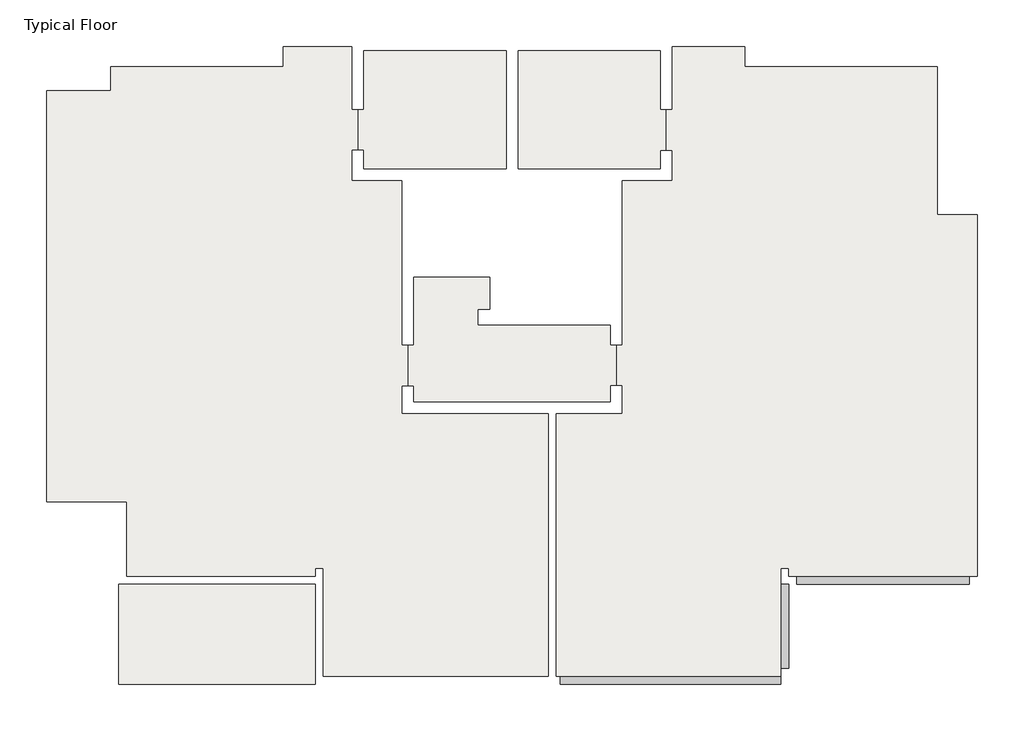
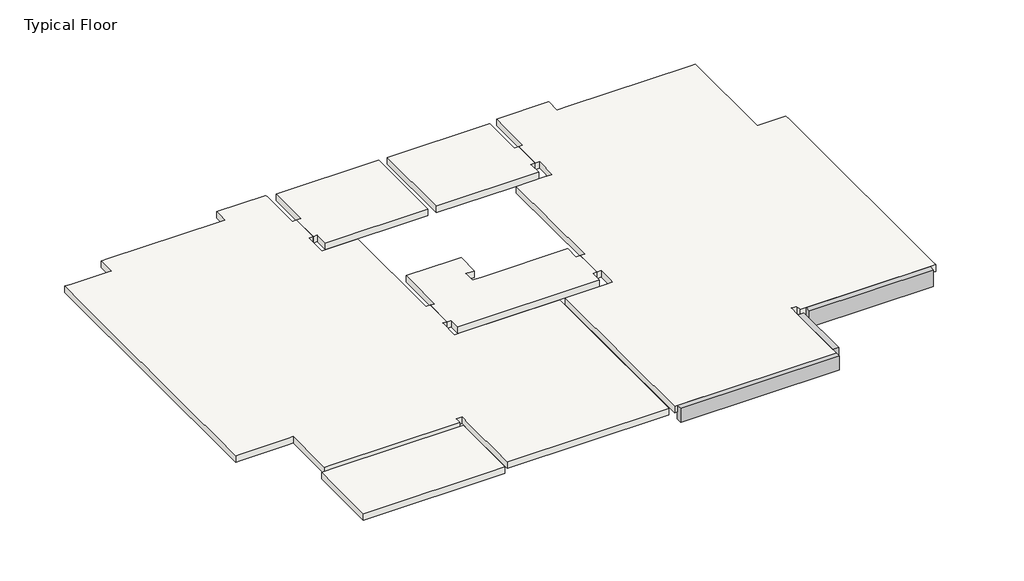
# One storey: 6 slabs, 3 beams.
"""IFC4 building model written with IfcOpenShell, lengths in millimetres."""

from ifc_helpers import new_model, si_unit, frame, origin, place, context, project, spatial, polyline, outline, extrude, faceted_brep, element, save

model = new_model("IFC4")

# Units and contexts
model_context = context("Model", 3, world=origin())
ifc_project = project(units=[si_unit("LENGTHUNIT", "METRE", prefix="MILLI")], contexts=[model_context])

# Site, building, storey
site = spatial("IfcSite", under=ifc_project)
building = spatial("IfcBuilding", under=site)
storey = spatial("IfcBuildingStorey", under=building, Name="Typical Floor", Elevation=3100.0)

# Beams
placement = place(None, origin())
element("IfcBeam", 1, ObjectType="Concrete Rectengular Beam : 20/50", at=placement, inside=storey, context=model_context, shape_type="Brep", body=[
    faceted_brep([(6304.7124885, -12504.8386239, 3100.0), (6304.7124885, -12304.8386239, 3100.0), (804.183388, -12304.8386239, 3100.0), (804.183388, -12504.8386239, 3100.0), (6304.7124885, -12304.8386239, 2860.0), (6304.7124885, -12304.8386239, 2600.0), (804.183388, -12304.8386239, 2600.0), (6304.7124885, -12504.8386239, 2600.0), (804.183388, -12504.8386239, 2600.0)], [[[0, 1, 2, 3]], [[1, 4, 5, 6, 2]], [[5, 7, 8, 6]], [[3, 8, 7, 0]], [[0, 7, 5, 4, 1]], [[3, 2, 6, 8]]]),
])
element("IfcBeam", 2, ObjectType="Concrete Rectengular Beam : 20/60", at=placement, inside=storey, context=model_context, shape_type="Brep", body=[
    faceted_brep([(6704.7124885, -9805.3677244, 3100.0), (6704.7124885, -10005.3677244, 3100.0), (11003.1251869, -10005.3677244, 3100.0), (11003.1251869, -9805.3677244, 3100.0), (6704.7124885, -10005.3677244, 2500.0), (11003.1251869, -10005.3677244, 2500.0), (6704.7124885, -9805.3677244, 2500.0), (11003.1251869, -9805.3677244, 2500.0), (11003.1251869, -9805.3677244, 2860.0), (6704.7124885, -9805.3677244, 2860.0)], [[[0, 1, 2, 3]], [[1, 4, 5, 2]], [[4, 6, 7, 5]], [[0, 3, 8, 7, 6, 9]], [[1, 0, 9, 6, 4]], [[3, 2, 5, 7, 8]]]),
])
element("IfcBeam", 3, ObjectType="Concrete Rectengular Beam : 20/60", at=placement, inside=storey, context=model_context, shape_type="Brep", body=[
    faceted_brep([(6304.7124885, -12104.8386239, 3100.0), (6504.7124885, -12104.8386239, 3100.0), (6504.7124885, -10005.3677244, 3100.0), (6304.7124885, -10005.3677244, 3100.0), (6504.7124885, -12104.8386239, 2500.0), (6504.7124885, -10005.3677244, 2500.0), (6304.7124885, -12104.8386239, 2500.0), (6304.7124885, -10005.3677244, 2500.0), (6304.7124885, -10005.3677244, 2860.0), (6304.7124885, -12104.8386239, 2860.0)], [[[0, 1, 2, 3]], [[1, 4, 5, 2]], [[4, 6, 7, 5]], [[0, 3, 8, 7, 6, 9]], [[1, 0, 9, 6, 4]], [[2, 5, 7, 8, 3]]]),
])

# Slabs
element("IfcSlab", 4, ObjectType="24", at=placement, inside=storey, context=model_context, shape_type="Brep", body=[
    faceted_brep([(2051.273335, -4056.1613752, 2860.0), (2201.273335, -4056.1613752, 2860.0), (2201.273335, -5055.6322747, 2860.0), (2053.3897372, -5055.6322747, 2860.0), (2053.3897372, -5455.6322747, 2860.0), (-2847.1393634, -5455.6322747, 2860.0), (-2847.1393634, -5057.2195763, 2860.0), (-2997.1393634, -5057.2195763, 2860.0), (-2997.1393634, -4056.1613752, 2860.0), (-2847.1393634, -4056.1613752, 2860.0), (-2847.1393634, -2356.6904757, 2860.0), (-1246.6102628, -2356.6904757, 2860.0), (-946.6102628, -2356.6904757, 2860.0), (-946.6102628, -3156.6904757, 2860.0), (-1246.6102628, -3156.6904757, 2860.0), (-1246.6102628, -3556.6904757, 2860.0), (-946.6102628, -3556.6904757, 2860.0), (2051.273335, -3556.6904757, 2860.0), (2201.273335, -4056.1613752, 3100.0), (2051.273335, -4056.1613752, 3100.0), (2051.273335, -3556.6904757, 3100.0), (-946.6102628, -3556.6904757, 3100.0), (-1246.6102628, -3556.6904757, 3100.0), (-1246.6102628, -3156.6904757, 3100.0), (-946.6102628, -3156.6904757, 3100.0), (-946.6102628, -2356.6904757, 3100.0), (-1246.6102628, -2356.6904757, 3100.0), (-2847.1393634, -2356.6904757, 3100.0), (-2847.1393634, -4056.1613752, 3100.0), (-2997.1393634, -4056.1613752, 3100.0), (-2997.1393634, -5057.2195763, 3100.0), (-2847.1393634, -5057.2195763, 3100.0), (-2847.1393634, -5455.6322747, 3100.0), (2053.3897372, -5455.6322747, 3100.0), (2053.3897372, -5055.6322747, 3100.0), (2201.273335, -5055.6322747, 3100.0)], [[[0, 1, 2, 3, 4, 5, 6, 7, 8, 9, 10, 11, 12, 13, 14, 15, 16, 17]], [[18, 19, 20, 21, 22, 23, 24, 25, 26, 27, 28, 29, 30, 31, 32, 33, 34, 35]], [[1, 0, 19, 18]], [[2, 1, 18, 35]], [[3, 2, 35, 34]], [[4, 3, 34, 33]], [[5, 4, 33, 32]], [[6, 5, 32, 31]], [[7, 6, 31, 30]], [[8, 7, 30, 29]], [[9, 8, 29, 28]], [[10, 9, 28, 27]], [[11, 10, 27, 26]], [[12, 11, 26, 25]], [[13, 12, 25, 24]], [[14, 13, 24, 23]], [[15, 14, 23, 22]], [[15, 22, 21, 20, 17, 16]], [[0, 17, 20, 19]]]),
])
element("IfcSlab", 5, ObjectType="24", at=placement, inside=storey, context=model_context, shape_type="SweptSolid", body=[
    extrude(outline(polyline([(3302.0669858, 3291.4576724), (3302.0669858, 1816.8544978), (3452.0669858, 1816.8544978), (3452.0669858, 811.5634925), (3302.0669858, 811.5634925), (3302.0669858, 343.3095243), (-246.0811623, 343.3095243), (-246.0811623, 3291.4576724), (3302.0669858, 3291.4576724)])), frame((0.0, 0.0, 2860.0), z_axis=(0.0, 0.0, 1.0), x_axis=(1.0, 0.0, 0.0)), (0.0, 0.0, 1.0), 240.0),
])
element("IfcSlab", 6, ObjectType="24", at=placement, inside=storey, context=model_context, shape_type="SweptSolid", body=[
    extrude(outline(polyline([(-546.0811623, 3291.4576724), (-546.0811623, 343.3095243), (-4095.816612, 343.3095243), (-4095.816612, 817.9126989), (-4245.816612, 817.9126989), (-4245.816612, 1816.8544978), (-4095.816612, 1816.8544978), (-4095.816612, 3291.4576724), (-546.0811623, 3291.4576724)])), frame((0.0, 0.0, 2860.0), z_axis=(0.0, 0.0, 1.0), x_axis=(1.0, 0.0, 0.0)), (0.0, 0.0, 1.0), 240.0),
])
element("IfcSlab", 7, ObjectType="24", at=placement, inside=storey, context=model_context, shape_type="Brep", body=[
    faceted_brep([(3452.0669858, 1816.8544978, 2860.0), (3602.0669858, 1816.8544978, 2860.0), (3602.0669858, 3291.4576724, 2860.0), (3602.0669858, 3391.4576724, 2860.0), (5403.1251869, 3391.4576724, 2860.0), (5403.1251869, 2891.9867729, 2860.0), (5803.1251869, 2891.9867729, 2860.0), (10002.0669858, 2891.9867729, 2860.0), (10202.0669858, 2891.9867729, 2860.0), (10202.0669858, 2691.9867729, 2860.0), (10202.0669858, -606.4259255, 2860.0), (10202.0669858, -806.4259255, 2860.0), (11203.1251869, -806.4259255, 2860.0), (11203.1251869, -9605.3677244, 2860.0), (11203.1251869, -9805.3677244, 2860.0), (11003.1251869, -9805.3677244, 2860.0), (6704.7124885, -9805.3677244, 2860.0), (6504.7124885, -9805.3677244, 2860.0), (6504.7124885, -9605.3677244, 2860.0), (6304.7124885, -9605.3677244, 2860.0), (6304.7124885, -10005.3677244, 2860.0), (6304.7124885, -12104.8386239, 2860.0), (6304.7124885, -12304.8386239, 2860.0), (804.183388, -12304.8386239, 2860.0), (704.183388, -12304.8386239, 2860.0), (704.183388, -12104.8386239, 2860.0), (704.183388, -5755.6322747, 2860.0), (2053.3897372, -5755.6322747, 2860.0), (2353.3897372, -5755.6322747, 2860.0), (2353.3897372, -5055.6322747, 2860.0), (2203.3897372, -5055.6322747, 2860.0), (2201.273335, -5055.6322747, 2860.0), (2201.273335, -4056.1613752, 2860.0), (2351.273335, -4056.1613752, 2860.0), (2351.273335, 43.3095243, 2860.0), (3302.0669858, 43.3095243, 2860.0), (3602.0669858, 43.3095243, 2860.0), (3602.0669858, 811.5634925, 2860.0), (3452.0669858, 811.5634925, 2860.0), (3602.0669858, 1816.8544978, 3100.0), (3452.0669858, 1816.8544978, 3100.0), (3452.0669858, 811.5634925, 3100.0), (3602.0669858, 811.5634925, 3100.0), (3602.0669858, 43.3095243, 3100.0), (3302.0669858, 43.3095243, 3100.0), (2351.273335, 43.3095243, 3100.0), (2351.273335, -4056.1613752, 3100.0), (2201.273335, -4056.1613752, 3100.0), (2201.273335, -5055.6322747, 3100.0), (2203.3897372, -5055.6322747, 3100.0), (2353.3897372, -5055.6322747, 3100.0), (2353.3897372, -5755.6322747, 3100.0), (2053.3897372, -5755.6322747, 3100.0), (704.183388, -5755.6322747, 3100.0), (704.183388, -9405.3677244, 3100.0), (704.183388, -10005.3677244, 3100.0), (704.183388, -12104.8386239, 3100.0), (704.183388, -12304.8386239, 3100.0), (804.183388, -12304.8386239, 3100.0), (6304.7124885, -12304.8386239, 3100.0), (6304.7124885, -12104.8386239, 3100.0), (6304.7124885, -10005.3677244, 3100.0), (6304.7124885, -9605.3677244, 3100.0), (6504.7124885, -9605.3677244, 3100.0), (6504.7124885, -9805.3677244, 3100.0), (6704.7124885, -9805.3677244, 3100.0), (11003.1251869, -9805.3677244, 3100.0), (11203.1251869, -9805.3677244, 3100.0), (11203.1251869, -9605.3677244, 3100.0), (11203.1251869, -5956.955026, 3100.0), (11203.1251869, -5306.955026, 3100.0), (11203.1251869, -1006.4259255, 3100.0), (11203.1251869, -806.4259255, 3100.0), (10202.0669858, -806.4259255, 3100.0), (10202.0669858, -606.4259255, 3100.0), (10202.0669858, 2691.9867729, 3100.0), (10202.0669858, 2891.9867729, 3100.0), (10002.0669858, 2891.9867729, 3100.0), (5803.1251869, 2891.9867729, 3100.0), (5403.1251869, 2891.9867729, 3100.0), (5403.1251869, 3391.4576724, 3100.0), (3602.0669858, 3391.4576724, 3100.0), (3602.0669858, 3291.4576724, 3100.0)], [[[0, 1, 2, 3, 4, 5, 6, 7, 8, 9, 10, 11, 12, 13, 14, 15, 16, 17, 18, 19, 20, 21, 22, 23, 24, 25, 26, 27, 28, 29, 30, 31, 32, 33, 34, 35, 36, 37, 38]], [[39, 40, 41, 42, 43, 44, 45, 46, 47, 48, 49, 50, 51, 52, 53, 54, 55, 56, 57, 58, 59, 60, 61, 62, 63, 64, 65, 66, 67, 68, 69, 70, 71, 72, 73, 74, 75, 76, 77, 78, 79, 80, 81, 82]], [[1, 0, 40, 39]], [[1, 39, 82, 81, 3, 2]], [[4, 3, 81, 80]], [[5, 4, 80, 79]], [[5, 79, 78, 77, 76, 8, 7, 6]], [[8, 76, 75, 74, 73, 11, 10, 9]], [[12, 11, 73, 72]], [[12, 72, 71, 70, 69, 68, 67, 14, 13]], [[14, 67, 66, 65, 64, 17, 16, 15]], [[18, 17, 64, 63]], [[19, 18, 63, 62]], [[20, 19, 62, 61]], [[20, 61, 60, 59, 22, 21]], [[22, 59, 58, 57, 24, 23]], [[24, 57, 56, 55, 54, 53, 26, 25]], [[26, 53, 52, 51, 28, 27]], [[29, 28, 51, 50]], [[30, 29, 50, 49]], [[31, 30, 49, 48]], [[32, 31, 48, 47]], [[33, 32, 47, 46]], [[34, 33, 46, 45]], [[34, 45, 44, 43, 36, 35]], [[37, 36, 43, 42]], [[38, 37, 42, 41]], [[0, 38, 41, 40]]]),
])
element("IfcSlab", 8, ObjectType="24", at=placement, inside=storey, context=model_context, shape_type="Brep", body=[
    faceted_brep([(-5097.4039136, -9605.3677244, 2860.0), (-5297.4039136, -9605.3677244, 2860.0), (-5297.4039136, -9805.3677244, 2860.0), (-5497.4039136, -9805.3677244, 2860.0), (-9695.2875115, -9805.3677244, 2860.0), (-9995.816612, -9805.3677244, 2860.0), (-9995.816612, -7955.6322747, 2860.0), (-10195.816612, -7955.6322747, 2860.0), (-11796.8748131, -7955.6322747, 2860.0), (-11996.8748131, -7955.6322747, 2860.0), (-11996.8748131, -7755.6322747, 2860.0), (-11996.8748131, 2091.9867729, 2860.0), (-11996.8748131, 2291.9867729, 2860.0), (-11796.8748131, 2291.9867729, 2860.0), (-10596.8748131, 2291.9867729, 2860.0), (-10396.8748131, 2291.9867729, 2860.0), (-10396.8748131, 2891.9867729, 2860.0), (-10196.8748131, 2891.9867729, 2860.0), (-6296.3457126, 2891.9867729, 2860.0), (-6096.3457126, 2891.9867729, 2860.0), (-6096.3457126, 3391.4576724, 2860.0), (-4395.816612, 3391.4576724, 2860.0), (-4395.816612, 3291.4576724, 2860.0), (-4395.816612, 1816.8544978, 2860.0), (-4245.816612, 1816.8544978, 2860.0), (-4245.816612, 817.9126989, 2860.0), (-4395.816612, 817.9126989, 2860.0), (-4395.816612, 343.3095243, 2860.0), (-4395.816612, 43.3095243, 2860.0), (-3147.1393634, 43.3095243, 2860.0), (-3147.1393634, -4056.1613752, 2860.0), (-2997.1393634, -4056.1613752, 2860.0), (-2997.1393634, -5057.2195763, 2860.0), (-3147.1393634, -5057.2195763, 2860.0), (-3147.1393634, -5755.6322747, 2860.0), (-2847.1393634, -5755.6322747, 2860.0), (504.183388, -5755.6322747, 2860.0), (504.183388, -12104.8386239, 2860.0), (504.183388, -12304.8386239, 2860.0), (404.183388, -12304.8386239, 2860.0), (-5097.4039136, -12304.8386239, 2860.0), (-5097.4039136, -12104.8386239, 2860.0), (-5097.4039136, -10005.3677244, 2860.0), (-5297.4039136, -9605.3677244, 3100.0), (-5097.4039136, -9605.3677244, 3100.0), (-5097.4039136, -10005.3677244, 3100.0), (-5097.4039136, -12104.8386239, 3100.0), (-5097.4039136, -12304.8386239, 3100.0), (404.183388, -12304.8386239, 3100.0), (504.183388, -12304.8386239, 3100.0), (504.183388, -12104.8386239, 3100.0), (504.183388, -10005.3677244, 3100.0), (504.183388, -9405.3677244, 3100.0), (504.183388, -5755.6322747, 3100.0), (-2847.1393634, -5755.6322747, 3100.0), (-3147.1393634, -5755.6322747, 3100.0), (-3147.1393634, -5057.2195763, 3100.0), (-2997.1393634, -5057.2195763, 3100.0), (-2997.1393634, -4056.1613752, 3100.0), (-3147.1393634, -4056.1613752, 3100.0), (-3147.1393634, 43.3095243, 3100.0), (-4395.816612, 43.3095243, 3100.0), (-4395.816612, 343.3095243, 3100.0), (-4395.816612, 817.9126989, 3100.0), (-4245.816612, 817.9126989, 3100.0), (-4245.816612, 1816.8544978, 3100.0), (-4395.816612, 1816.8544978, 3100.0), (-4395.816612, 3291.4576724, 3100.0), (-4395.816612, 3391.4576724, 3100.0), (-6096.3457126, 3391.4576724, 3100.0), (-6096.3457126, 2891.9867729, 3100.0), (-6296.3457126, 2891.9867729, 3100.0), (-10196.8748131, 2891.9867729, 3100.0), (-10396.8748131, 2891.9867729, 3100.0), (-10396.8748131, 2291.9867729, 3100.0), (-10596.8748131, 2291.9867729, 3100.0), (-11796.8748131, 2291.9867729, 3100.0), (-11996.8748131, 2291.9867729, 3100.0), (-11996.8748131, 2091.9867729, 3100.0), (-11996.8748131, -407.4841265, 3100.0), (-11996.8748131, -807.4841265, 3100.0), (-11996.8748131, -3806.4259255, 3100.0), (-11996.8748131, -4456.4259255, 3100.0), (-11996.8748131, -7755.6322747, 3100.0), (-11996.8748131, -7955.6322747, 3100.0), (-11796.8748131, -7955.6322747, 3100.0), (-10195.816612, -7955.6322747, 3100.0), (-9995.816612, -7955.6322747, 3100.0), (-9995.816612, -9805.3677244, 3100.0), (-9695.2875115, -9805.3677244, 3100.0), (-5497.4039136, -9805.3677244, 3100.0), (-5297.4039136, -9805.3677244, 3100.0)], [[[0, 1, 2, 3, 4, 5, 6, 7, 8, 9, 10, 11, 12, 13, 14, 15, 16, 17, 18, 19, 20, 21, 22, 23, 24, 25, 26, 27, 28, 29, 30, 31, 32, 33, 34, 35, 36, 37, 38, 39, 40, 41, 42]], [[43, 44, 45, 46, 47, 48, 49, 50, 51, 52, 53, 54, 55, 56, 57, 58, 59, 60, 61, 62, 63, 64, 65, 66, 67, 68, 69, 70, 71, 72, 73, 74, 75, 76, 77, 78, 79, 80, 81, 82, 83, 84, 85, 86, 87, 88, 89, 90, 91]], [[47, 40, 39, 38, 49, 48]], [[40, 47, 46, 45, 44, 0, 42, 41]], [[1, 0, 44, 43]], [[2, 1, 43, 91]], [[2, 91, 90, 89, 88, 5, 4, 3]], [[6, 5, 88, 87]], [[6, 87, 86, 85, 84, 9, 8, 7]], [[9, 84, 83, 82, 81, 80, 79, 78, 77, 12, 11, 10]], [[12, 77, 76, 75, 74, 15, 14, 13]], [[16, 15, 74, 73]], [[16, 73, 72, 71, 70, 19, 18, 17]], [[20, 19, 70, 69]], [[21, 20, 69, 68]], [[21, 68, 67, 66, 23, 22]], [[24, 23, 66, 65]], [[25, 24, 65, 64]], [[26, 25, 64, 63]], [[26, 63, 62, 61, 28, 27]], [[29, 28, 61, 60]], [[30, 29, 60, 59]], [[31, 30, 59, 58]], [[32, 31, 58, 57]], [[33, 32, 57, 56]], [[34, 33, 56, 55]], [[34, 55, 54, 53, 36, 35]], [[36, 53, 52, 51, 50, 49, 38, 37]]]),
])
element("IfcSlab", 9, ObjectType="24", at=placement, inside=storey, context=model_context, shape_type="Brep", body=[
    faceted_brep([(-5297.4039136, -10005.3677244, 2860.0), (-5297.4039136, -12504.8386239, 2860.0), (-10195.816612, -12504.8386239, 2860.0), (-10195.816612, -10005.3677244, 2860.0), (-5297.4039136, -12504.8386239, 3100.0), (-5297.4039136, -12104.8386239, 3100.0), (-5297.4039136, -10005.3677244, 3100.0), (-5497.4039136, -10005.3677244, 3100.0), (-9695.2875115, -10005.3677244, 3100.0), (-10195.816612, -10005.3677244, 3100.0), (-10195.816612, -12504.8386239, 3100.0)], [[[0, 1, 2, 3]], [[4, 5, 6, 7, 8, 9, 10]], [[1, 0, 6, 5, 4]], [[2, 1, 4, 10]], [[3, 2, 10, 9]], [[0, 3, 9, 8, 7, 6]]]),
])

save(model, "model.ifc")

# Revit data of these elements
# Type "Concrete Rectengular Beam : 20/50"
#   Length [instance default] = 152.4 cm
#   b = 20 cm
#   h = 50 cm
#   Structural Material [instance default] = Concrete
#   Assembly Code = ""
# Type "Concrete Rectengular Beam : 20/60"
#   Length [instance default] = 152.4 cm
#   b = 20 cm
#   h = 60 cm
#   Structural Material [instance default] = Concrete
#   Assembly Code = ""
# Type "24"
#   Function = 0
#   Layers, outside or top first: 24 cm "Concrete" (function 1)
# Element 1 (IfcBeam, "Concrete Rectengular Beam : 20/50")
#   Comments = ""
#   Mark = "B8"
#   SOFiSTiK_AMG_Comments = ""
#   SOFiSTiK_AMG_Scheduled = yes
#   SOFiSTiK_AMG_Adjusted = yes
#   Structural Material = Concrete
#   Phase Created = New Construction
#   Materials on its faces: "Concrete"
# Element 2 (IfcBeam, "Concrete Rectengular Beam : 20/60")
#   Comments = ""
#   Mark = "B19"
#   SOFiSTiK_AMG_Comments = ""
#   SOFiSTiK_AMG_Scheduled = yes
#   SOFiSTiK_AMG_Adjusted = yes
#   Structural Material = Concrete
#   Phase Created = New Construction
#   Materials on its faces: "Concrete"
# Element 3 (IfcBeam, "Concrete Rectengular Beam : 20/60")
#   Comments = ""
#   Mark = "B20"
#   SOFiSTiK_AMG_Comments = ""
#   SOFiSTiK_AMG_Scheduled = yes
#   SOFiSTiK_AMG_Adjusted = yes
#   Structural Material = Concrete
#   Phase Created = New Construction
#   Materials on its faces: "Concrete"
# Element 4 (IfcSlab, "24")
#   Mark = "S1"
#   SOFiSTiK_AMG_Comments = ""
#   built-in parameter 1001955 = -1.5708 (stored number, unit not read)
#   Height Offset From Level = 0 cm
#   built-in parameter 1001954 = 1
#   SOFiSTiK_AMG_Scheduled = yes
#   SOFiSTiK_AMG_Adjusted = yes
#   Phase Created = New Construction
#   Materials on its faces: "Concrete"
# Element 5 (IfcSlab, "24")
#   Mark = "S2"
#   SOFiSTiK_AMG_Comments = ""
#   Height Offset From Level = 0 cm
#   built-in parameter 1001954 = 1
#   SOFiSTiK_AMG_Scheduled = yes
#   SOFiSTiK_AMG_Adjusted = yes
#   Phase Created = New Construction
#   Materials on its faces: "Concrete"
# Element 6 (IfcSlab, "24")
#   Mark = "S3"
#   SOFiSTiK_AMG_Comments = ""
#   Height Offset From Level = 0 cm
#   built-in parameter 1001954 = 1
#   SOFiSTiK_AMG_Scheduled = yes
#   SOFiSTiK_AMG_Adjusted = yes
#   Phase Created = New Construction
#   Materials on its faces: "Concrete"
# Element 7 (IfcSlab, "24")
#   Mark = "S4"
#   SOFiSTiK_AMG_Comments = ""
#   built-in parameter 1001955 = 1.5708 (stored number, unit not read)
#   Height Offset From Level = 0 cm
#   built-in parameter 1001954 = 1
#   SOFiSTiK_AMG_Scheduled = yes
#   SOFiSTiK_AMG_Adjusted = no
#   Phase Created = New Construction
#   Materials on its faces: "Concrete"
# Element 8 (IfcSlab, "24")
#   Mark = "S5"
#   SOFiSTiK_AMG_Comments = ""
#   Height Offset From Level = 0 cm
#   built-in parameter 1001954 = 1
#   SOFiSTiK_AMG_Scheduled = yes
#   SOFiSTiK_AMG_Adjusted = yes
#   Phase Created = New Construction
#   Materials on its faces: "Concrete"
# Element 9 (IfcSlab, "24")
#   Mark = "S6"
#   SOFiSTiK_AMG_Comments = ""
#   Height Offset From Level = 0 cm
#   built-in parameter 1001954 = 1
#   SOFiSTiK_AMG_Scheduled = yes
#   SOFiSTiK_AMG_Adjusted = yes
#   Phase Created = New Construction
#   Materials on its faces: "Concrete"
# Materials
#   "Concrete": class "Concrete", colour RGB 192 192 192, transparency 0, Keynote = "01000", Description = "Cast-in-place concrete", Cost = 0
